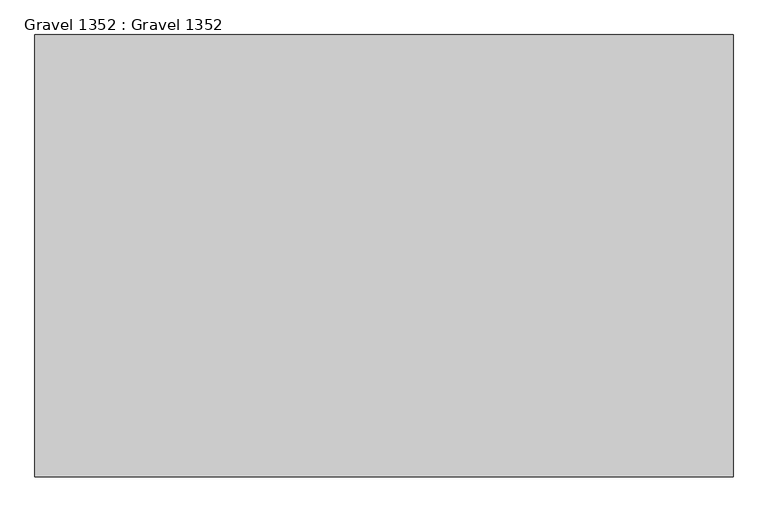
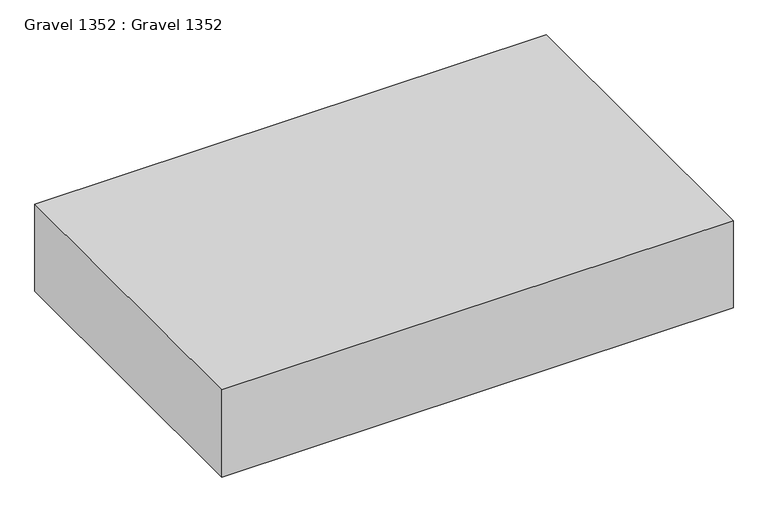
"""IFC4 building model written with IfcOpenShell, lengths in millimetres: proxy geometry, Gravel 1352 : Gravel 1352."""

from ifc_helpers import new_model, si_unit, frame, origin, place, context, project, spatial, polyline, outline, extrude, source, transform, mapped, element, save


def gravel_1352_gravel_1352_b5835376(model_context):
    return source(origin(), model_context, "Body", "SweptSolid", [
        extrude(outline(polyline([(3694.2883192, 9730.3375834), (3694.2883192, 10997.0939628), (5694.2883192, 10997.0939628), (5694.2883192, 9730.3375834), (3694.2883192, 9730.3375834)])), frame((0.0, 0.0, 35744.9946418), z_axis=(0.0, 0.0, 1.0), x_axis=(1.0, 0.0, 0.0)), (0.0, 0.0, 1.0), 360.4577188),
    ])


if __name__ == "__main__":
    model = new_model("IFC4")
    model_context = context("Model", 3, world=origin())
    ifc_project = project(units=[si_unit("LENGTHUNIT", "METRE", prefix="MILLI")], contexts=[model_context])
    site = spatial("IfcSite", under=ifc_project)
    building = spatial("IfcBuilding", under=site)
    placement = place(None, origin())
    gravel_1352_gravel_1352_shape = gravel_1352_gravel_1352_b5835376(model_context)
    element("IfcBuildingElementProxy", 1, Name="Gravel 1352 : Gravel 1352", ObjectType="Gravel 1352 : Gravel 1352", at=placement, inside=building, context=model_context, shape_type="MappedRepresentation", body=[
        mapped(gravel_1352_gravel_1352_shape, transform((0.0, 0.0, 0.0), x_axis=(1.0, 0.0, 0.0), y_axis=(0.0, 1.0, 0.0), z_axis=(0.0, 0.0, 1.0))),
    ])
    save(model, "model.ifc")

# Revit data of these elements
# Type "Gravel 1352 : Gravel 1352"
#   NameOverride = "Gravel"
# Element 1 (IfcBuildingElementProxy, "Gravel 1352 : Gravel 1352")
#   Materials on its faces: "4\" MIN. CRUSHED GRAVEL (NO FINES)"
# Materials
#   "4\" MIN. CRUSHED GRAVEL (NO FINES)": class "Unassigned", colour RGB 145 162 188, transparency 0, Cost = 0
